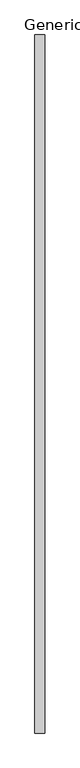
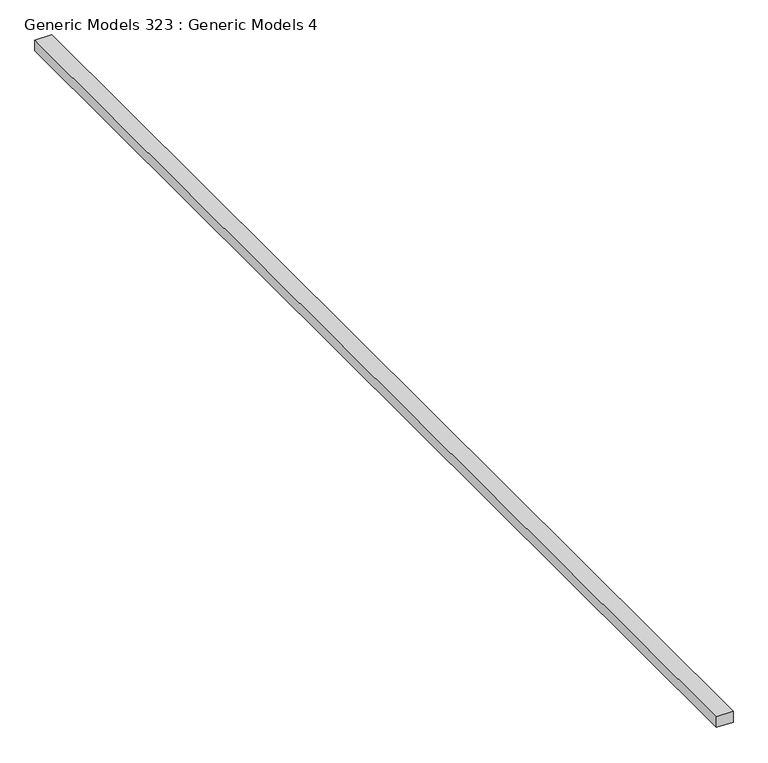
"""IFC4 building model written with IfcOpenShell, lengths in millimetres: proxy geometry, Generic Models 323 : Generic Models 4."""

from ifc_helpers import new_model, si_unit, frame, origin, place, context, project, spatial, polyline, outline, extrude, source, transform, mapped, element, save


def generic_models_323_generic_models_4_9d793d27(model_context):
    return source(origin(), model_context, "Body", "SweptSolid", [
        extrude(outline(polyline([(123716.9153984, 8750.1263705), (123716.9153984, 8572.3263705), (123602.9610056, 8572.3263705), (123594.5880456, 8750.1263705), (123716.9153984, 8750.1263705)])), frame((0.0, -5493.3230338, 0.0), z_axis=(0.0, 1.0, 0.0), x_axis=(0.0, 0.0, 1.0)), (0.0, 0.0, 1.0), 12547.6),
    ])


if __name__ == "__main__":
    model = new_model("IFC4")
    model_context = context("Model", 3, world=origin())
    ifc_project = project(units=[si_unit("LENGTHUNIT", "METRE", prefix="MILLI")], contexts=[model_context])
    site = spatial("IfcSite", under=ifc_project)
    building = spatial("IfcBuilding", under=site)
    placement = place(None, origin())
    generic_models_323_generic_models_4_shape = generic_models_323_generic_models_4_9d793d27(model_context)
    element("IfcBuildingElementProxy", 1, Name="Generic Models 323 : Generic Models 4", ObjectType="Generic Models 323 : Generic Models 4", at=placement, inside=building, context=model_context, shape_type="MappedRepresentation", body=[
        mapped(generic_models_323_generic_models_4_shape, transform((0.0, 0.0, 0.0), x_axis=(1.0, 0.0, 0.0), y_axis=(0.0, 1.0, 0.0), z_axis=(0.0, 0.0, 1.0))),
    ])
    save(model, "model.ifc")

# Revit data of these elements
# Element 1 (IfcBuildingElementProxy, "Generic Models 323 : Generic Models 4")
#   Materials on its faces: "_LANDSCAPING STONE T.B.D."
# Materials
#   "_LANDSCAPING STONE T.B.D.": class "Generic", colour RGB 122 131 148, transparency 0, Cost = 0
